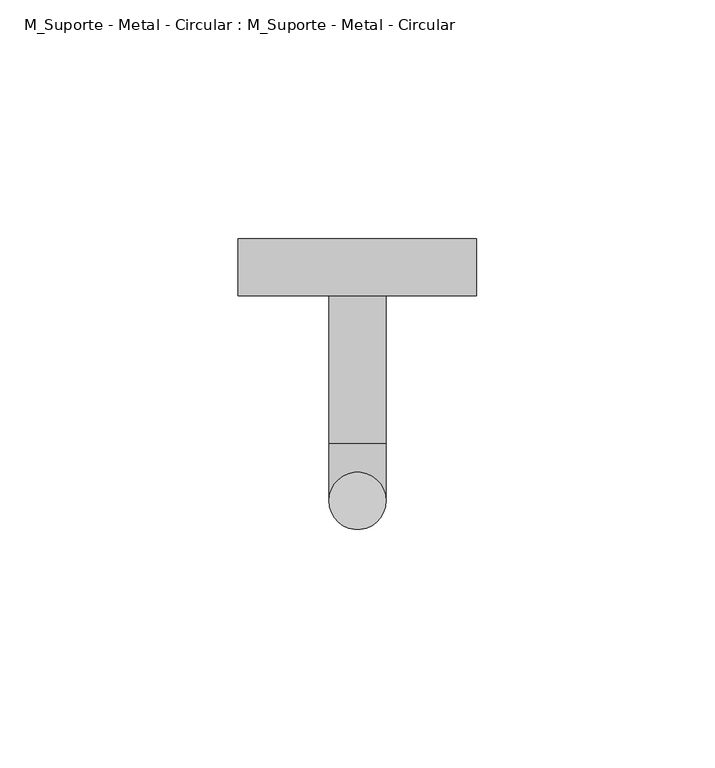
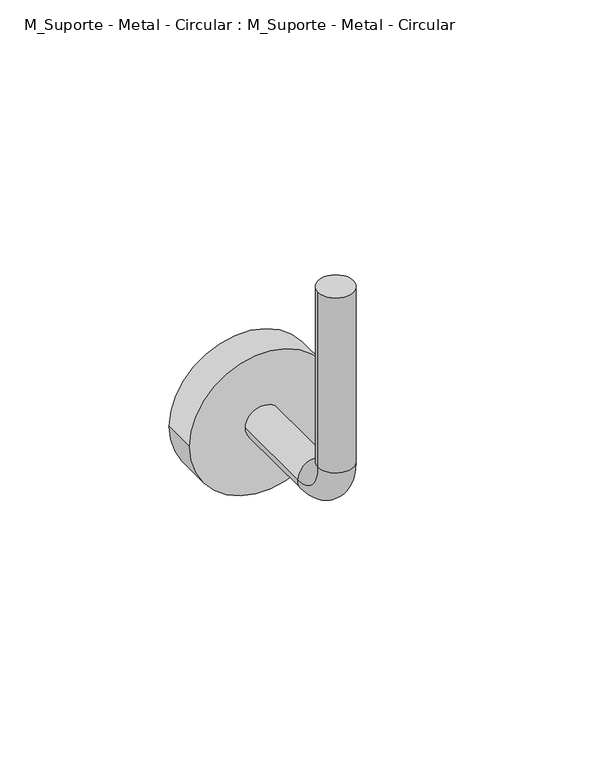
"""IFC4 building model written with IfcOpenShell, lengths in millimetres: proxy geometry, M_Suporte - Metal - Circular : M_Suporte - Metal - Circular."""

from ifc_helpers import new_model, si_unit, point, frame, frame_2d, origin, origin_with_axes, place, context, project, spatial, circle_curve, ellipse_curve, trimmed, segment, composite_curve, outline, extrude, source, transform, mapped, element, save
from ifc_brep_helpers import plane_surface, cylinder_surface, revolved_surface, advanced_brep


def m_suporte_metal_circular_m_suporte_metal_circular_cf76aa7a(model_context):
    return source(origin(), model_context, "Body", "SolidModel", [
        advanced_brep(
        [(-6.0, 0.0, 0.0), (6.0, 0.0, 0.0), (-6.0, 0.0, -63.0), (6.0, 0.0, -63.0), (6.0, 12.0, -75.0), (-6.0, 12.0, -75.0), (-6.0, 43.0, -75.0), (6.0, 43.0, -75.0)],
        [
            (0, 1, circle_curve(origin_with_axes(), 6.0)),
            (1, 0, circle_curve(origin_with_axes(), 6.0)),
            (0, 2),
            (2, 3, circle_curve(frame((0.0, 0.0, -63.0), z_axis=(0.0, 0.0, 1.0), x_axis=(1.0, 0.0, 0.0)), 6.0)),
            (3, 1),
            (3, 2, circle_curve(frame((0.0, 0.0, -63.0), z_axis=(0.0, 0.0, 1.0), x_axis=(1.0, 0.0, 0.0)), 6.0)),
            (4, 3, circle_curve(frame((6.0, 12.0, -63.0), z_axis=(-1.0, 0.0, 0.0), x_axis=(0.0, -1.0, 0.0)), 12.0)),
            (2, 5, circle_curve(frame((-6.0, 12.0, -63.0), z_axis=(1.0, 0.0, 0.0), x_axis=(0.0, -1.0, 0.0)), 12.0)),
            (5, 4, circle_curve(frame((0.0, 12.0, -75.0), z_axis=(0.0, -1.0, 0.0), x_axis=(1.0, 0.0, 0.0)), 6.0)),
            (4, 5, circle_curve(frame((0.0, 12.0, -75.0), z_axis=(0.0, -1.0, 0.0), x_axis=(1.0, 0.0, 0.0)), 6.0)),
            (6, 7, circle_curve(frame((0.0, 43.0, -75.0), z_axis=(0.0, 1.0, 0.0), x_axis=(1.0, 0.0, 0.0)), 6.0)),
            (7, 6, circle_curve(frame((0.0, 43.0, -75.0), z_axis=(0.0, 1.0, 0.0), x_axis=(1.0, 0.0, 0.0)), 6.0)),
            (5, 6),
            (7, 4),
        ],
        [
            plane_surface(origin_with_axes()),
            cylinder_surface(origin_with_axes(), 6.0),
            revolved_surface(trimmed(ellipse_curve(frame((0.0, 0.0, -63.0), z_axis=(0.0, 0.0, 1.0), x_axis=(1.0, 0.0, 0.0)), 6.0, 6.0), [point((-6.0, 0.0, -63.0))], [point((6.0, 0.0, -63.0))], True, "CARTESIAN"), (0.0, 12.0, -63.0), (1.0, 0.0, 0.0)),
            revolved_surface(trimmed(ellipse_curve(frame((0.0, 0.0, -63.0), z_axis=(0.0, 0.0, 1.0), x_axis=(1.0, 0.0, 0.0)), 6.0, 6.0), [point((6.0, 0.0, -63.0))], [point((-6.0, 0.0, -63.0))], True, "CARTESIAN"), (0.0, 12.0, -63.0), (1.0, 0.0, 0.0)),
            plane_surface(frame((0.0, 43.0, -75.0), z_axis=(0.0, 1.0, 0.0), x_axis=(1.0, 0.0, 0.0))),
            cylinder_surface(frame((0.0, 12.0, -75.0), z_axis=(0.0, -1.0, 0.0), x_axis=(1.0, 0.0, 0.0)), 6.0),
        ],
        [
            (0, [[1, 2]]),
            (1, [[-1, 3, 4, 5]]),
            (1, [[-2, -5, 6, -3]]),
            (2, [[7, -4, 8, 9]]),
            (3, [[-8, -6, -7, 10]]),
            (4, [[11, 12]]),
            (5, [[-9, 13, -12, 14]]),
            (5, [[-10, -14, -11, -13]]),
        ],
    ),
        extrude(outline(composite_curve([segment(trimmed(circle_curve(frame_2d((-75.0, 0.0)), 25.0), [point((-75.0, -25.0))], [point((-75.0, 25.0))], False, "CARTESIAN"), True, "CONTINUOUS"), segment(trimmed(circle_curve(frame_2d((-75.0, 0.0)), 25.0), [point((-75.0, 25.0))], [point((-75.0, -25.0))], False, "CARTESIAN"), True, "CONTINUOUS")], self_intersect=False)), frame((0.0, 43.0, 0.0), z_axis=(0.0, 1.0, 0.0), x_axis=(0.0, 0.0, 1.0)), (0.0, 0.0, 1.0), 12.0),
    ])


if __name__ == "__main__":
    model = new_model("IFC4")
    model_context = context("Model", 3, world=origin())
    ifc_project = project(units=[si_unit("LENGTHUNIT", "METRE", prefix="MILLI")], contexts=[model_context])
    site = spatial("IfcSite", under=ifc_project)
    building = spatial("IfcBuilding", under=site)
    placement = place(None, origin())
    m_suporte_metal_circular_m_suporte_metal_circular_shape = m_suporte_metal_circular_m_suporte_metal_circular_cf76aa7a(model_context)
    element("IfcBuildingElementProxy", 1, Name="M_Suporte - Metal - Circular : M_Suporte - Metal - Circular", ObjectType="M_Suporte - Metal - Circular : M_Suporte - Metal - Circular", at=placement, inside=building, context=model_context, shape_type="MappedRepresentation", body=[
        mapped(m_suporte_metal_circular_m_suporte_metal_circular_shape, transform((0.0, 0.0, 0.0), x_axis=(1.0, 0.0, 0.0), y_axis=(0.0, 1.0, 0.0), z_axis=(0.0, 0.0, 1.0))),
    ])
    save(model, "model.ifc")

# Revit data of these elements
# Type "M_Suporte - Metal - Circular : M_Suporte - Metal - Circular"
#   T1 = 0.012 m
#   Raio 2 = 0.006 m
#   Raio 1 = 0.025 m
#   built-in parameter 1152166 = 0.246063 (stored number, unit not read)
#   built-in parameter 1152165 [instance default] = 0.246063 (stored number, unit not read)
#   Raio da curva = 0.012 m
#   Material de suporte = none
# Element 1 (IfcBuildingElementProxy, "M_Suporte - Metal - Circular : M_Suporte - Metal - Circular")
#   built-in parameter 1152165 = 0.180446 (stored number, unit not read)
